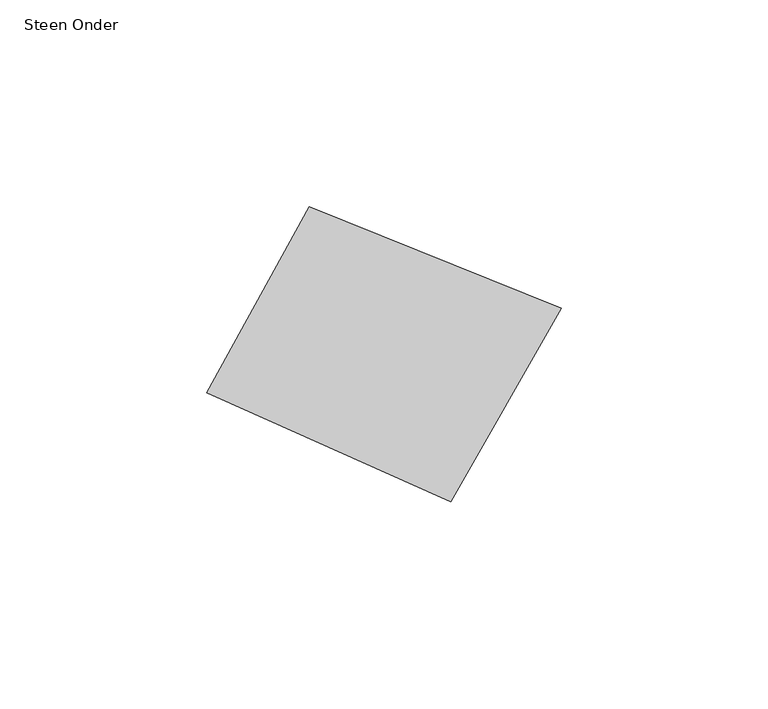
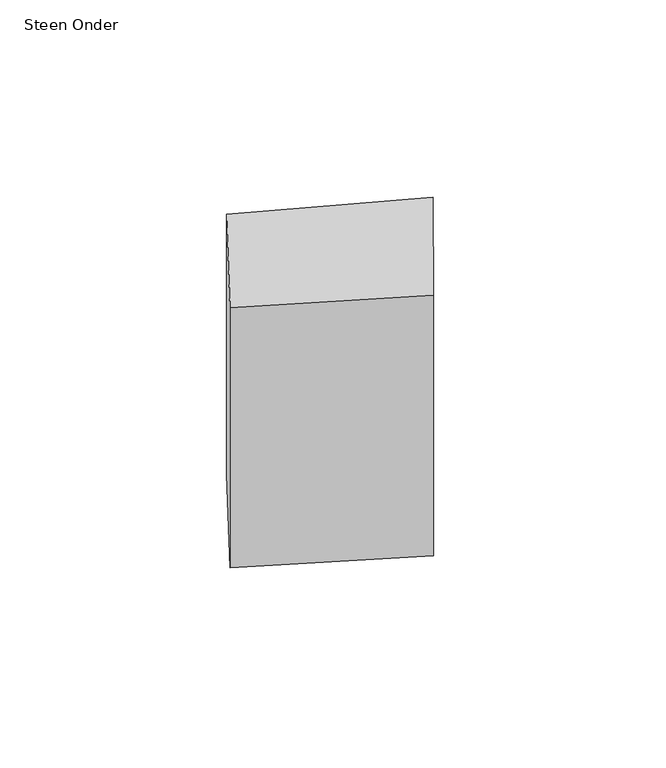
"""IFC4 building model written with IfcOpenShell, lengths in millimetres: proxy geometry, 00_GMA_steen_versie_4 : Steen Onder."""

from ifc_helpers import new_model, si_unit, frame, origin, place, context, project, spatial, polyline, outline, extrude, source, transform, mapped, element, save


def steen_onder_f442e5d6(model_context):
    return source(origin(), model_context, "Body", "SweptSolid", [
        extrude(outline(polyline([(131.2649037, 52.8706917), (104.5973844, 6.1260635), (45.6641138, 32.4887), (70.4039345, 77.4217363), (131.2649037, 52.8706917)])), frame((0.0, 0.0, -100.0), z_axis=(0.0, 0.0, 1.0), x_axis=(1.0, 0.0, 0.0)), (0.0, 0.0, 1.0), 100.0),
    ])


if __name__ == "__main__":
    model = new_model("IFC4")
    model_context = context("Model", 3, world=origin())
    ifc_project = project(units=[si_unit("LENGTHUNIT", "METRE", prefix="MILLI")], contexts=[model_context])
    site = spatial("IfcSite", under=ifc_project)
    building = spatial("IfcBuilding", under=site)
    placement = place(None, origin())
    steen_onder_shape = steen_onder_f442e5d6(model_context)
    element("IfcBuildingElementProxy", 1, Name="00_GMA_steen_versie_4 : Steen Onder", ObjectType="00_GMA_steen_versie_4 : Steen Onder", at=placement, inside=building, context=model_context, shape_type="MappedRepresentation", body=[
        mapped(steen_onder_shape, transform((0.0, 0.0, 0.0), x_axis=(1.0, 0.0, 0.0), y_axis=(0.0, 1.0, 0.0), z_axis=(0.0, 0.0, 1.0))),
    ])
    save(model, "model.ifc")

# Revit data of these elements
# Type "00_GMA_steen_versie_4 : Steen Onder"
#   StootVoegHalfBoven [instance default] = 5 mm
#   StootVoegHalf [instance default] = 5 mm
#   StootVoegBreedteOnder = 10 mm
#   StootVoegBreedteBoven = 10 mm
#   Steendikte = 100 mm
#   LintVoegOnderHalf = 0 mm
#   LintVoegOnder = 0 mm
#   LintVoegBovenHalf = 5 mm
#   LintVoegBoven = 10 mm
#   materiaal = none
#   MateriaalVoeg = none
#   Default Elevation = 0
